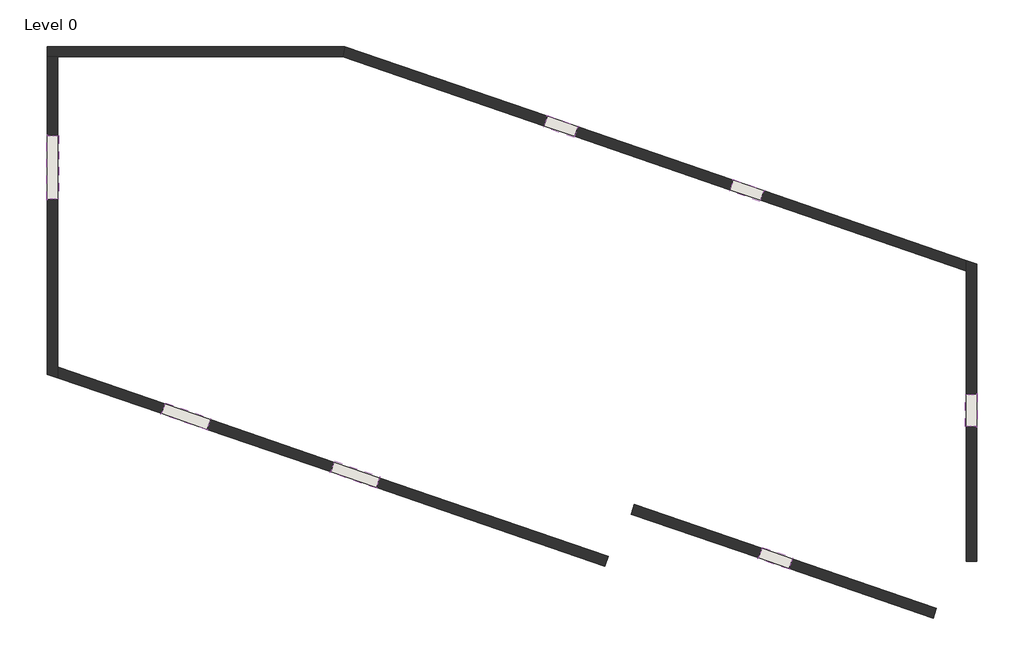
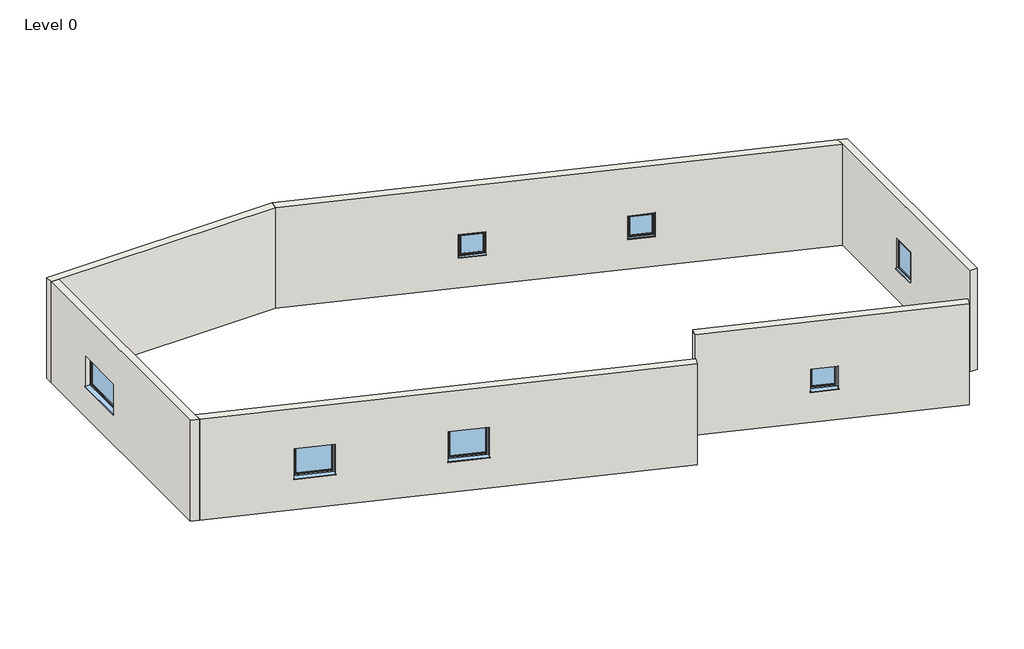
# One storey: 7 windows, 6 walls.
"""IFC4 building model written with IfcOpenShell, lengths in millimetres."""

import ifcopenshell
import ifcopenshell.guid

model = None  # the IFC model being written
_history = None  # IfcOwnerHistory: only IFC2X3 demands one
_inside = {}  # id of a spatial element -> (the spatial element, [elements in it])
_under = {}  # id of a project, library or spatial element -> (it, [spatial elements below it])
_declared = {}  # id of a project -> (the project, [libraries it declares])
_typed = {}  # id of a type object -> (the type object, [elements of that type])
_made_of = {}  # id of a material, layer set ... -> (it, [elements and type objects made of it])


def new_model(schema):
    """Start an empty IFC model of exactly this schema.

    Asked for "IFC4X3", IfcOpenShell would pick the latest addendum, in which some entities
    have other attributes; the version numbers below select the first issue.
    IFC2X3 requires an IfcOwnerHistory on every rooted entity: one is made here for all.
    """
    global model, _history
    if schema == "IFC4X3":
        model = ifcopenshell.file(schema_version=(4, 3, 0, 0))
    else:
        model = ifcopenshell.file(schema=schema)
    _inside.clear()
    _under.clear()
    _declared.clear()
    _typed.clear()
    _made_of.clear()
    _history = None
    if model.schema == "IFC2X3":
        org = make("IfcOrganization", Name="unknown")
        user = make(
            "IfcPersonAndOrganization",
            ThePerson=make("IfcPerson", FamilyName="unknown"),
            TheOrganization=org,
        )
        app = make(
            "IfcApplication",
            ApplicationDeveloper=org,
            Version="unknown",
            ApplicationFullName="unknown",
            ApplicationIdentifier="unknown",
        )
        _history = make(
            "IfcOwnerHistory",
            OwningUser=user,
            OwningApplication=app,
            ChangeAction="ADDED",
            CreationDate=0,
        )
    return model


def make(cls, **values):
    """One entity of the class cls with the attributes given. An attribute that is None is left unset."""
    return model.create_entity(
        cls, **{name: value for name, value in values.items() if value is not None}
    )


def rooted(cls, **values):
    """An entity with a GlobalId (a new one), such as an element, a storey or a relation."""
    return make(cls, GlobalId=ifcopenshell.guid.new(), OwnerHistory=_history, **values)


def si_unit(unit_type, name, prefix=None):
    """IfcSIUnit, for example si_unit("LENGTHUNIT", "METRE", prefix="MILLI")."""
    return make("IfcSIUnit", UnitType=unit_type, Prefix=prefix, Name=name)


def assignment(units):
    """IfcUnitAssignment: the units of a project."""
    return None if units is None else make("IfcUnitAssignment", Units=units)


def point(xyz):
    """IfcCartesianPoint."""
    return None if xyz is None else make("IfcCartesianPoint", Coordinates=xyz)


def direction(xyz):
    """IfcDirection."""
    return None if xyz is None else make("IfcDirection", DirectionRatios=xyz)


def frame(location, z_axis=None, x_axis=None):
    """IfcAxis2Placement3D, a coordinate frame: its origin and axes. An axis left out is left unset."""
    return make(
        "IfcAxis2Placement3D",
        Location=point(location),
        Axis=direction(z_axis),
        RefDirection=direction(x_axis),
    )


def origin():
    """The frame at (0, 0, 0) with its axes left unset."""
    return frame((0.0, 0.0, 0.0))


def place(relative_to, where):
    """IfcLocalPlacement: puts the frame where relative to a parent placement (None: the world)."""
    return make(
        "IfcLocalPlacement", PlacementRelTo=relative_to, RelativePlacement=where
    )


def context(
    kind, dimensions, precision=None, world=None, true_north=None, identifier=None
):
    """IfcGeometricRepresentationContext, for example the 3D "Model" context."""
    return make(
        "IfcGeometricRepresentationContext",
        ContextIdentifier=identifier,
        ContextType=kind,
        CoordinateSpaceDimension=dimensions,
        Precision=precision,
        WorldCoordinateSystem=world,
        TrueNorth=true_north,
    )


def project(units=None, contexts=None):
    """IfcProject with its units and contexts."""
    return rooted(
        "IfcProject",
        Name="project",
        RepresentationContexts=contexts,
        UnitsInContext=assignment(units),
    )


def spatial(cls, under=None, at=None, **own):
    """A site, building, storey or space (cls), placed at a placement, below another one or the project."""
    s = rooted(cls, ObjectPlacement=at, **own)
    if under is not None:
        _under.setdefault(under.id(), (under, []))[1].append(s)
    return s


def polyline(points):
    """IfcPolyline through the points."""
    return make("IfcPolyline", Points=[point(p) for p in points])


def outline(outer, holes=None, kind="AREA"):
    """IfcArbitraryClosedProfileDef: a profile drawn as a closed curve; with holes, ...WithVoids."""
    if holes is None:
        return make("IfcArbitraryClosedProfileDef", ProfileType=kind, OuterCurve=outer)
    return make(
        "IfcArbitraryProfileDefWithVoids",
        ProfileType=kind,
        OuterCurve=outer,
        InnerCurves=holes,
    )


def extrude(swept, where, along, depth):
    """IfcExtrudedAreaSolid: the profile swept, set in the frame where, extruded along a direction by depth."""
    return make(
        "IfcExtrudedAreaSolid",
        SweptArea=swept,
        Position=where,
        ExtrudedDirection=direction(along),
        Depth=depth,
    )


def faces_of(points, faces, orient=None, outer=None):
    """IfcFace entities. A face is a list of loops; a loop is a list of indices into points, from 0.

    orient and outer hold one flag for each loop. By default every Orientation is true, the
    first loop of a face is its IfcFaceOuterBound and the others are IfcFaceBound.
    """
    made = []
    for i, loops in enumerate(faces):
        bounds = []
        for j, loop in enumerate(loops):
            is_outer = j == 0 if outer is None else outer[i][j]
            bounds.append(
                make(
                    "IfcFaceOuterBound" if is_outer else "IfcFaceBound",
                    Bound=make("IfcPolyLoop", Polygon=[points[k] for k in loop]),
                    Orientation=True if orient is None else orient[i][j],
                )
            )
        made.append(make("IfcFace", Bounds=bounds))
    return made


def faceted_brep(points, faces, orient=None, outer=None, voids=None):
    """IfcFacetedBrep: a solid bounded by flat faces; with voids (closed shells), ...WithVoids."""
    shared = [point(p) for p in points]
    hull = make("IfcClosedShell", CfsFaces=faces_of(shared, faces, orient, outer))
    if voids is None:
        return make("IfcFacetedBrep", Outer=hull)
    return make(
        "IfcFacetedBrepWithVoids",
        Outer=hull,
        Voids=[
            make(cls, CfsFaces=faces_of(shared, fs, o, b)) for cls, fs, o, b in voids
        ],
    )


def shape(context_of_items, identifier, shape_type, items):
    """IfcShapeRepresentation: the items that make up one representation, for example the "Body"."""
    return make(
        "IfcShapeRepresentation",
        ContextOfItems=context_of_items,
        RepresentationIdentifier=identifier,
        RepresentationType=shape_type,
        Items=items,
    )


def source(mapping_origin, context_of_items, identifier, shape_type, items):
    """IfcRepresentationMap: a shape defined once, which mapped items show again and again."""
    return make(
        "IfcRepresentationMap",
        MappingOrigin=mapping_origin,
        MappedRepresentation=shape(context_of_items, identifier, shape_type, items),
    )


def transform(
    local_origin,
    x_axis=None,
    y_axis=None,
    z_axis=None,
    scale=None,
    scale2=None,
    scale3=None,
    uniform=True,
):
    """IfcCartesianTransformationOperator3D, or its non-uniform kind. x_axis, y_axis, z_axis: its Axis1, 2, 3."""
    if uniform:
        return make(
            "IfcCartesianTransformationOperator3D",
            Axis1=direction(x_axis),
            Axis2=direction(y_axis),
            LocalOrigin=point(local_origin),
            Scale=scale,
            Axis3=direction(z_axis),
        )
    return make(
        "IfcCartesianTransformationOperator3DnonUniform",
        Axis1=direction(x_axis),
        Axis2=direction(y_axis),
        LocalOrigin=point(local_origin),
        Scale=scale,
        Axis3=direction(z_axis),
        Scale2=scale2,
        Scale3=scale3,
    )


def mapped(mapping_source, mapping_target):
    """IfcMappedItem: shows the shape of a source again, moved by a transform."""
    return make(
        "IfcMappedItem", MappingSource=mapping_source, MappingTarget=mapping_target
    )


def made_of(thing, what):
    """Note that an element or type object is made of a material, layer set ...; save() writes the relation."""
    if what is not None:
        _made_of.setdefault(what.id(), (what, []))[1].append(thing)
    return thing


def element(
    cls,
    number,
    at=None,
    inside=None,
    cuts=None,
    type_object=None,
    material=None,
    context=None,
    identifier="Body",
    shape_type=None,
    held_by="IfcProductDefinitionShape",
    body=None,
    shapes=None,
    **own,
):
    """One element of the class cls, such as IfcWall. Its Tag is "e" and its number.

    at: its placement. inside: the storey or other place that contains it. cuts: it is an
    opening in that element (IfcRelVoidsElement). A single representation is given by context,
    identifier, shape_type and body (its items); several are given by shapes. held_by: the class
    of the entity that holds the representations. save() writes the other relations.
    """
    e = rooted(cls, Tag="e%d" % number, ObjectPlacement=at, **own)
    if body is not None:
        shapes = [shape(context, identifier, shape_type, body)]
    if shapes is not None:
        e.Representation = make(held_by, Representations=shapes)
    if inside is not None:
        _inside.setdefault(inside.id(), (inside, []))[1].append(e)
    if cuts is not None:
        rooted(
            "IfcRelVoidsElement", RelatingBuildingElement=cuts, RelatedOpeningElement=e
        )
    if type_object is not None:
        _typed.setdefault(type_object.id(), (type_object, []))[1].append(e)
    return made_of(e, material)


def aggregate(whole, parts):
    """IfcRelAggregates: a whole, such as a stair, and the parts it consists of."""
    return rooted("IfcRelAggregates", RelatingObject=whole, RelatedObjects=parts)


def save(model, path):
    """Write the relations noted so far, then the file.

    IfcRelAggregates (storeys below a building ...), IfcRelContainedInSpatialStructure (elements
    in a storey), IfcRelDefinesByType, IfcRelAssociatesMaterial and IfcRelDeclares: one each for
    every whole, place, type object, material and project.
    """
    for whole, parts in _under.values():
        aggregate(whole, parts)
    for where, things in _inside.values():
        rooted(
            "IfcRelContainedInSpatialStructure",
            RelatedElements=things,
            RelatingStructure=where,
        )
    for kind, things in _typed.values():
        rooted("IfcRelDefinesByType", RelatedObjects=things, RelatingType=kind)
    for what, things in _made_of.values():
        rooted("IfcRelAssociatesMaterial", RelatedObjects=things, RelatingMaterial=what)
    for by, libraries in _declared.values():
        rooted("IfcRelDeclares", RelatingContext=by, RelatedDefinitions=libraries)
    model.write(path)


def windows_sgl_plain_1360x1210mm_d0b87b97(model_context):
    return source(origin(), model_context, "Body", "SolidModel", [
        extrude(outline(polyline([(-705.0, -161.5434322), (-705.0, -136.5434322), (-680.0, -136.5434322), (-680.0, 20.4565678), (680.0, 20.4565678), (680.0, -136.5434322), (705.0, -136.5434322), (705.0, -161.5434322), (-705.0, -161.5434322)])), frame((0.0, 0.0, 900.0), z_axis=(0.0, 0.0, 1.0), x_axis=(1.0, 0.0, 0.0)), (0.0, 0.0, 1.0), 25.0),
        faceted_brep([(-680.0, 20.4565678, 900.0), (680.0, 20.4565678, 900.0), (680.0, 20.4565678, 2110.0), (-680.0, 20.4565678, 2110.0), (-620.0, 20.4565678, 2050.0), (620.0, 20.4565678, 2050.0), (620.0, 20.4565678, 975.0), (-620.0, 20.4565678, 975.0), (-680.0, 103.4565678, 2110.0), (-680.0, 103.4565678, 951.0), (-680.0, 118.4565678, 949.68767), (-680.0, 118.4565678, 944.7449676), (-680.0, 190.9565678, 933.8088847), (-680.0, 190.9565678, 900.0), (680.0, 103.4565678, 2110.0), (680.0, 103.4565678, 951.0), (-640.0, 103.4565678, 2070.0), (-640.0, 103.4565678, 963.0), (640.0, 103.4565678, 963.0), (640.0, 103.4565678, 2070.0), (-640.0, 38.4565678, 2070.0), (-640.0, 38.4565678, 963.0), (640.0, 38.4565678, 2070.0), (640.0, 38.4565678, 963.0), (-620.0, 38.4565678, 2050.0), (-620.0, 38.4565678, 975.0), (620.0, 38.4565678, 975.0), (620.0, 38.4565678, 2050.0), (680.0, 190.9565678, 900.0), (680.0, 190.9565678, 933.8088847), (680.0, 118.4565678, 944.7449676), (680.0, 118.4565678, 949.68767)], [[[0, 1, 2, 3], [4, 5, 6, 7]], [[0, 3, 8, 9, 10, 11, 12, 13]], [[9, 8, 14, 15], [16, 17, 18, 19]], [[17, 16, 20, 21]], [[20, 22, 23, 21], [24, 25, 26, 27]], [[24, 4, 7, 25]], [[3, 2, 14, 8]], [[16, 19, 22, 20]], [[5, 4, 24, 27]], [[15, 14, 2, 1, 28, 29, 30, 31]], [[19, 18, 23, 22]], [[5, 27, 26, 6]], [[28, 1, 0, 13]], [[29, 28, 13, 12]], [[30, 29, 12, 11]], [[31, 30, 11, 10]], [[15, 31, 10, 9]], [[21, 23, 18, 17]], [[7, 6, 26, 25]]]),
        extrude(outline(polyline([(610.0, 67.4565678), (-610.0, 67.4565678), (-610.0, 91.4565678), (610.0, 91.4565678), (610.0, 67.4565678)])), frame((0.0, 0.0, 993.0), z_axis=(0.0, 0.0, 1.0), x_axis=(1.0, 0.0, 0.0)), (0.0, 0.0, 1.0), 1047.0),
        faceted_brep([(-650.0, 103.4565678, 2080.0), (-650.0, 109.2300705, 2080.0), (-650.0, 109.2300705, 953.0), (-650.0, 103.4565678, 953.0), (-640.0, 38.4565678, 2070.0), (-640.0, 103.4565678, 2070.0), (-640.0, 103.4565678, 963.0), (-640.0, 38.4565678, 963.0), (-600.0, 52.9494677, 2030.0), (-610.1480377, 38.4565678, 2040.1480377), (-610.1480377, 38.4565678, 992.8519623), (-600.0, 52.9494677, 1003.0), (-600.0, 67.4565678, 2030.0), (-600.0, 67.4565678, 1003.0), (-610.0, 91.4565678, 2040.0), (-610.0, 67.4565678, 2040.0), (-610.0, 67.4565678, 993.0), (-610.0, 91.4565678, 993.0), (-600.0, 109.2300705, 2030.0), (-600.0, 91.4565678, 2030.0), (-600.0, 91.4565678, 1003.0), (-600.0, 109.2300705, 1003.0), (-617.4457548, 115.0035732, 2047.4457548), (-617.4457548, 115.0035732, 985.5542452), (-639.2153903, 115.0035732, 2069.2153903), (-639.2153903, 115.0035732, 963.7846097), (650.0, 109.2300705, 953.0), (650.0, 103.4565678, 953.0), (640.0, 103.4565678, 963.0), (640.0, 38.4565678, 963.0), (610.1480377, 38.4565678, 992.8519623), (600.0, 52.9494677, 1003.0), (600.0, 67.4565678, 1003.0), (610.0, 67.4565678, 993.0), (610.0, 91.4565678, 993.0), (600.0, 91.4565678, 1003.0), (600.0, 109.2300705, 1003.0), (617.4457548, 115.0035732, 985.5542452), (639.2153903, 115.0035732, 963.7846097), (650.0, 109.2300705, 2080.0), (650.0, 103.4565678, 2080.0), (640.0, 103.4565678, 2070.0), (640.0, 38.4565678, 2070.0), (610.1480377, 38.4565678, 2040.1480377), (600.0, 52.9494677, 2030.0), (600.0, 67.4565678, 2030.0), (610.0, 67.4565678, 2040.0), (610.0, 91.4565678, 2040.0), (600.0, 91.4565678, 2030.0), (600.0, 109.2300705, 2030.0), (617.4457548, 115.0035732, 2047.4457548), (639.2153903, 115.0035732, 2069.2153903)], [[[0, 1, 2, 3]], [[4, 5, 6, 7]], [[8, 9, 10, 11]], [[12, 8, 11, 13]], [[14, 15, 16, 17]], [[18, 19, 20, 21]], [[22, 18, 21, 23]], [[1, 24, 25, 2]], [[3, 2, 26, 27]], [[7, 6, 28, 29]], [[11, 10, 30, 31]], [[13, 11, 31, 32]], [[17, 16, 33, 34]], [[21, 20, 35, 36]], [[23, 21, 36, 37]], [[2, 25, 38, 26]], [[27, 26, 39, 40]], [[29, 28, 41, 42]], [[31, 30, 43, 44]], [[32, 31, 44, 45]], [[34, 33, 46, 47]], [[36, 35, 48, 49]], [[37, 36, 49, 50]], [[26, 38, 51, 39]], [[40, 39, 1, 0]], [[3, 27, 40, 0], [5, 41, 28, 6]], [[42, 41, 5, 4]], [[7, 29, 42, 4], [9, 43, 30, 10]], [[44, 43, 9, 8]], [[45, 44, 8, 12]], [[15, 46, 33, 16], [13, 32, 45, 12]], [[47, 46, 15, 14]], [[17, 34, 47, 14], [19, 48, 35, 20]], [[49, 48, 19, 18]], [[50, 49, 18, 22]], [[24, 51, 38, 25], [23, 37, 50, 22]], [[39, 51, 24, 1]]]),
    ])


def windows_sgl_plain_1810x1210mm_114720e4(model_context):
    return source(origin(), model_context, "Body", "SolidModel", [
        extrude(outline(polyline([(-930.0, -161.5434322), (-930.0, -136.5434322), (-905.0, -136.5434322), (-905.0, 20.4565678), (905.0, 20.4565678), (905.0, -136.5434322), (930.0, -136.5434322), (930.0, -161.5434322), (-930.0, -161.5434322)])), frame((0.0, 0.0, 900.0), z_axis=(0.0, 0.0, 1.0), x_axis=(1.0, 0.0, 0.0)), (0.0, 0.0, 1.0), 25.0),
        faceted_brep([(-905.0, 20.4565678, 900.0), (905.0, 20.4565678, 900.0), (905.0, 20.4565678, 2110.0), (-905.0, 20.4565678, 2110.0), (-845.0, 20.4565678, 2050.0), (845.0, 20.4565678, 2050.0), (845.0, 20.4565678, 975.0), (-845.0, 20.4565678, 975.0), (-905.0, 103.4565678, 2110.0), (-905.0, 103.4565678, 951.0), (-905.0, 118.4565678, 949.68767), (-905.0, 118.4565678, 944.7449676), (-905.0, 190.9565678, 933.8088847), (-905.0, 190.9565678, 900.0), (905.0, 103.4565678, 2110.0), (905.0, 103.4565678, 951.0), (-865.0, 103.4565678, 2070.0), (-865.0, 103.4565678, 963.0), (865.0, 103.4565678, 963.0), (865.0, 103.4565678, 2070.0), (-865.0, 38.4565678, 2070.0), (-865.0, 38.4565678, 963.0), (865.0, 38.4565678, 2070.0), (865.0, 38.4565678, 963.0), (-845.0, 38.4565678, 2050.0), (-845.0, 38.4565678, 975.0), (845.0, 38.4565678, 975.0), (845.0, 38.4565678, 2050.0), (905.0, 190.9565678, 900.0), (905.0, 190.9565678, 933.8088847), (905.0, 118.4565678, 944.7449676), (905.0, 118.4565678, 949.68767)], [[[0, 1, 2, 3], [4, 5, 6, 7]], [[0, 3, 8, 9, 10, 11, 12, 13]], [[9, 8, 14, 15], [16, 17, 18, 19]], [[17, 16, 20, 21]], [[20, 22, 23, 21], [24, 25, 26, 27]], [[24, 4, 7, 25]], [[3, 2, 14, 8]], [[16, 19, 22, 20]], [[5, 4, 24, 27]], [[15, 14, 2, 1, 28, 29, 30, 31]], [[19, 18, 23, 22]], [[5, 27, 26, 6]], [[28, 1, 0, 13]], [[29, 28, 13, 12]], [[30, 29, 12, 11]], [[31, 30, 11, 10]], [[15, 31, 10, 9]], [[21, 23, 18, 17]], [[7, 6, 26, 25]]]),
        extrude(outline(polyline([(835.0, 67.4565678), (-835.0, 67.4565678), (-835.0, 91.4565678), (835.0, 91.4565678), (835.0, 67.4565678)])), frame((0.0, 0.0, 993.0), z_axis=(0.0, 0.0, 1.0), x_axis=(1.0, 0.0, 0.0)), (0.0, 0.0, 1.0), 1047.0),
        faceted_brep([(-875.0, 103.4565678, 2080.0), (-875.0, 109.2300705, 2080.0), (-875.0, 109.2300705, 953.0), (-875.0, 103.4565678, 953.0), (-865.0, 38.4565678, 2070.0), (-865.0, 103.4565678, 2070.0), (-865.0, 103.4565678, 963.0), (-865.0, 38.4565678, 963.0), (-825.0, 52.9494677, 2030.0), (-835.1480377, 38.4565678, 2040.1480377), (-835.1480377, 38.4565678, 992.8519623), (-825.0, 52.9494677, 1003.0), (-825.0, 67.4565678, 2030.0), (-825.0, 67.4565678, 1003.0), (-835.0, 91.4565678, 2040.0), (-835.0, 67.4565678, 2040.0), (-835.0, 67.4565678, 993.0), (-835.0, 91.4565678, 993.0), (-825.0, 109.2300705, 2030.0), (-825.0, 91.4565678, 2030.0), (-825.0, 91.4565678, 1003.0), (-825.0, 109.2300705, 1003.0), (-842.4457548, 115.0035732, 2047.4457548), (-842.4457548, 115.0035732, 985.5542452), (-864.2153903, 115.0035732, 2069.2153903), (-864.2153903, 115.0035732, 963.7846097), (875.0, 109.2300705, 953.0), (875.0, 103.4565678, 953.0), (865.0, 103.4565678, 963.0), (865.0, 38.4565678, 963.0), (835.1480377, 38.4565678, 992.8519623), (825.0, 52.9494677, 1003.0), (825.0, 67.4565678, 1003.0), (835.0, 67.4565678, 993.0), (835.0, 91.4565678, 993.0), (825.0, 91.4565678, 1003.0), (825.0, 109.2300705, 1003.0), (842.4457548, 115.0035732, 985.5542452), (864.2153903, 115.0035732, 963.7846097), (875.0, 109.2300705, 2080.0), (875.0, 103.4565678, 2080.0), (865.0, 103.4565678, 2070.0), (865.0, 38.4565678, 2070.0), (835.1480377, 38.4565678, 2040.1480377), (825.0, 52.9494677, 2030.0), (825.0, 67.4565678, 2030.0), (835.0, 67.4565678, 2040.0), (835.0, 91.4565678, 2040.0), (825.0, 91.4565678, 2030.0), (825.0, 109.2300705, 2030.0), (842.4457548, 115.0035732, 2047.4457548), (864.2153903, 115.0035732, 2069.2153903)], [[[0, 1, 2, 3]], [[4, 5, 6, 7]], [[8, 9, 10, 11]], [[12, 8, 11, 13]], [[14, 15, 16, 17]], [[18, 19, 20, 21]], [[22, 18, 21, 23]], [[1, 24, 25, 2]], [[3, 2, 26, 27]], [[7, 6, 28, 29]], [[11, 10, 30, 31]], [[13, 11, 31, 32]], [[17, 16, 33, 34]], [[21, 20, 35, 36]], [[23, 21, 36, 37]], [[2, 25, 38, 26]], [[27, 26, 39, 40]], [[29, 28, 41, 42]], [[31, 30, 43, 44]], [[32, 31, 44, 45]], [[34, 33, 46, 47]], [[36, 35, 48, 49]], [[37, 36, 49, 50]], [[26, 38, 51, 39]], [[40, 39, 1, 0]], [[3, 27, 40, 0], [5, 41, 28, 6]], [[42, 41, 5, 4]], [[7, 29, 42, 4], [9, 43, 30, 10]], [[44, 43, 9, 8]], [[45, 44, 8, 12]], [[15, 46, 33, 16], [13, 32, 45, 12]], [[47, 46, 15, 14]], [[17, 34, 47, 14], [19, 48, 35, 20]], [[49, 48, 19, 18]], [[50, 49, 18, 22]], [[24, 51, 38, 25], [23, 37, 50, 22]], [[39, 51, 24, 1]]]),
    ])


def windows_sgl_plain_910x1210mm_58c8e711(model_context):
    return source(origin(), model_context, "Body", "SolidModel", [
        extrude(outline(polyline([(-480.0, -161.5434322), (-480.0, -136.5434322), (-455.0, -136.5434322), (-455.0, 20.4565678), (455.0, 20.4565678), (455.0, -136.5434322), (480.0, -136.5434322), (480.0, -161.5434322), (-480.0, -161.5434322)])), frame((0.0, 0.0, 900.0), z_axis=(0.0, 0.0, 1.0), x_axis=(1.0, 0.0, 0.0)), (0.0, 0.0, 1.0), 25.0),
        faceted_brep([(-455.0, 20.4565678, 900.0), (455.0, 20.4565678, 900.0), (455.0, 20.4565678, 2110.0), (-455.0, 20.4565678, 2110.0), (-395.0, 20.4565678, 2050.0), (395.0, 20.4565678, 2050.0), (395.0, 20.4565678, 975.0), (-395.0, 20.4565678, 975.0), (-455.0, 103.4565678, 2110.0), (-455.0, 103.4565678, 951.0), (-455.0, 118.4565678, 949.68767), (-455.0, 118.4565678, 944.7449676), (-455.0, 190.9565678, 933.8088847), (-455.0, 190.9565678, 900.0), (455.0, 103.4565678, 2110.0), (455.0, 103.4565678, 951.0), (-415.0, 103.4565678, 2070.0), (-415.0, 103.4565678, 963.0), (415.0, 103.4565678, 963.0), (415.0, 103.4565678, 2070.0), (-415.0, 38.4565678, 2070.0), (-415.0, 38.4565678, 963.0), (415.0, 38.4565678, 2070.0), (415.0, 38.4565678, 963.0), (-395.0, 38.4565678, 2050.0), (-395.0, 38.4565678, 975.0), (395.0, 38.4565678, 975.0), (395.0, 38.4565678, 2050.0), (455.0, 190.9565678, 900.0), (455.0, 190.9565678, 933.8088847), (455.0, 118.4565678, 944.7449676), (455.0, 118.4565678, 949.68767)], [[[0, 1, 2, 3], [4, 5, 6, 7]], [[0, 3, 8, 9, 10, 11, 12, 13]], [[9, 8, 14, 15], [16, 17, 18, 19]], [[17, 16, 20, 21]], [[20, 22, 23, 21], [24, 25, 26, 27]], [[24, 4, 7, 25]], [[3, 2, 14, 8]], [[16, 19, 22, 20]], [[5, 4, 24, 27]], [[15, 14, 2, 1, 28, 29, 30, 31]], [[19, 18, 23, 22]], [[5, 27, 26, 6]], [[28, 1, 0, 13]], [[29, 28, 13, 12]], [[30, 29, 12, 11]], [[31, 30, 11, 10]], [[15, 31, 10, 9]], [[21, 23, 18, 17]], [[7, 6, 26, 25]]]),
        extrude(outline(polyline([(385.0, 67.4565678), (-385.0, 67.4565678), (-385.0, 91.4565678), (385.0, 91.4565678), (385.0, 67.4565678)])), frame((0.0, 0.0, 993.0), z_axis=(0.0, 0.0, 1.0), x_axis=(1.0, 0.0, 0.0)), (0.0, 0.0, 1.0), 1047.0),
        faceted_brep([(-425.0, 103.4565678, 2080.0), (-425.0, 109.2300705, 2080.0), (-425.0, 109.2300705, 953.0), (-425.0, 103.4565678, 953.0), (-415.0, 38.4565678, 2070.0), (-415.0, 103.4565678, 2070.0), (-415.0, 103.4565678, 963.0), (-415.0, 38.4565678, 963.0), (-375.0, 52.9494677, 2030.0), (-385.1480377, 38.4565678, 2040.1480377), (-385.1480377, 38.4565678, 992.8519623), (-375.0, 52.9494677, 1003.0), (-375.0, 67.4565678, 2030.0), (-375.0, 67.4565678, 1003.0), (-385.0, 91.4565678, 2040.0), (-385.0, 67.4565678, 2040.0), (-385.0, 67.4565678, 993.0), (-385.0, 91.4565678, 993.0), (-375.0, 109.2300705, 2030.0), (-375.0, 91.4565678, 2030.0), (-375.0, 91.4565678, 1003.0), (-375.0, 109.2300705, 1003.0), (-392.4457548, 115.0035732, 2047.4457548), (-392.4457548, 115.0035732, 985.5542452), (-414.2153903, 115.0035732, 2069.2153903), (-414.2153903, 115.0035732, 963.7846097), (425.0, 109.2300705, 953.0), (425.0, 103.4565678, 953.0), (415.0, 103.4565678, 963.0), (415.0, 38.4565678, 963.0), (385.1480377, 38.4565678, 992.8519623), (375.0, 52.9494677, 1003.0), (375.0, 67.4565678, 1003.0), (385.0, 67.4565678, 993.0), (385.0, 91.4565678, 993.0), (375.0, 91.4565678, 1003.0), (375.0, 109.2300705, 1003.0), (392.4457548, 115.0035732, 985.5542452), (414.2153903, 115.0035732, 963.7846097), (425.0, 109.2300705, 2080.0), (425.0, 103.4565678, 2080.0), (415.0, 103.4565678, 2070.0), (415.0, 38.4565678, 2070.0), (385.1480377, 38.4565678, 2040.1480377), (375.0, 52.9494677, 2030.0), (375.0, 67.4565678, 2030.0), (385.0, 67.4565678, 2040.0), (385.0, 91.4565678, 2040.0), (375.0, 91.4565678, 2030.0), (375.0, 109.2300705, 2030.0), (392.4457548, 115.0035732, 2047.4457548), (414.2153903, 115.0035732, 2069.2153903)], [[[0, 1, 2, 3]], [[4, 5, 6, 7]], [[8, 9, 10, 11]], [[12, 8, 11, 13]], [[14, 15, 16, 17]], [[18, 19, 20, 21]], [[22, 18, 21, 23]], [[1, 24, 25, 2]], [[3, 2, 26, 27]], [[7, 6, 28, 29]], [[11, 10, 30, 31]], [[13, 11, 31, 32]], [[17, 16, 33, 34]], [[21, 20, 35, 36]], [[23, 21, 36, 37]], [[2, 25, 38, 26]], [[27, 26, 39, 40]], [[29, 28, 41, 42]], [[31, 30, 43, 44]], [[32, 31, 44, 45]], [[34, 33, 46, 47]], [[36, 35, 48, 49]], [[37, 36, 49, 50]], [[26, 38, 51, 39]], [[40, 39, 1, 0]], [[3, 27, 40, 0], [5, 41, 28, 6]], [[42, 41, 5, 4]], [[7, 29, 42, 4], [9, 43, 30, 10]], [[44, 43, 9, 8]], [[45, 44, 8, 12]], [[15, 46, 33, 16], [13, 32, 45, 12]], [[47, 46, 15, 14]], [[17, 34, 47, 14], [19, 48, 35, 20]], [[49, 48, 19, 18]], [[50, 49, 18, 22]], [[24, 51, 38, 25], [23, 37, 50, 22]], [[39, 51, 24, 1]]]),
    ])


def windows_sgl_plain_910x910mm_b9caa461(model_context):
    return source(origin(), model_context, "Body", "SolidModel", [
        extrude(outline(polyline([(-480.0, -161.5434322), (-480.0, -136.5434322), (-455.0, -136.5434322), (-455.0, 20.4565678), (455.0, 20.4565678), (455.0, -136.5434322), (480.0, -136.5434322), (480.0, -161.5434322), (-480.0, -161.5434322)])), frame((0.0, 0.0, 1200.0), z_axis=(0.0, 0.0, 1.0), x_axis=(1.0, 0.0, 0.0)), (0.0, 0.0, 1.0), 25.0),
        faceted_brep([(-455.0, 20.4565678, 1200.0), (455.0, 20.4565678, 1200.0), (455.0, 20.4565678, 2110.0), (-455.0, 20.4565678, 2110.0), (-395.0, 20.4565678, 2050.0), (395.0, 20.4565678, 2050.0), (395.0, 20.4565678, 1275.0), (-395.0, 20.4565678, 1275.0), (-455.0, 103.4565678, 2110.0), (-455.0, 103.4565678, 1251.0), (-455.0, 118.4565678, 1249.68767), (-455.0, 118.4565678, 1244.7449676), (-455.0, 190.9565678, 1233.8088847), (-455.0, 190.9565678, 1200.0), (455.0, 103.4565678, 2110.0), (455.0, 103.4565678, 1251.0), (-415.0, 103.4565678, 2070.0), (-415.0, 103.4565678, 1263.0), (415.0, 103.4565678, 1263.0), (415.0, 103.4565678, 2070.0), (-415.0, 38.4565678, 2070.0), (-415.0, 38.4565678, 1263.0), (415.0, 38.4565678, 2070.0), (415.0, 38.4565678, 1263.0), (-395.0, 38.4565678, 2050.0), (-395.0, 38.4565678, 1275.0), (395.0, 38.4565678, 1275.0), (395.0, 38.4565678, 2050.0), (455.0, 190.9565678, 1200.0), (455.0, 190.9565678, 1233.8088847), (455.0, 118.4565678, 1244.7449676), (455.0, 118.4565678, 1249.68767)], [[[0, 1, 2, 3], [4, 5, 6, 7]], [[0, 3, 8, 9, 10, 11, 12, 13]], [[9, 8, 14, 15], [16, 17, 18, 19]], [[17, 16, 20, 21]], [[20, 22, 23, 21], [24, 25, 26, 27]], [[24, 4, 7, 25]], [[3, 2, 14, 8]], [[16, 19, 22, 20]], [[5, 4, 24, 27]], [[15, 14, 2, 1, 28, 29, 30, 31]], [[19, 18, 23, 22]], [[5, 27, 26, 6]], [[28, 1, 0, 13]], [[29, 28, 13, 12]], [[30, 29, 12, 11]], [[31, 30, 11, 10]], [[15, 31, 10, 9]], [[21, 23, 18, 17]], [[7, 6, 26, 25]]]),
        extrude(outline(polyline([(385.0, 67.4565678), (-385.0, 67.4565678), (-385.0, 91.4565678), (385.0, 91.4565678), (385.0, 67.4565678)])), frame((0.0, 0.0, 1293.0), z_axis=(0.0, 0.0, 1.0), x_axis=(1.0, 0.0, 0.0)), (0.0, 0.0, 1.0), 747.0),
        faceted_brep([(-425.0, 103.4565678, 2080.0), (-425.0, 109.2300705, 2080.0), (-425.0, 109.2300705, 1253.0), (-425.0, 103.4565678, 1253.0), (-415.0, 38.4565678, 2070.0), (-415.0, 103.4565678, 2070.0), (-415.0, 103.4565678, 1263.0), (-415.0, 38.4565678, 1263.0), (-375.0, 52.9494677, 2030.0), (-385.1480377, 38.4565678, 2040.1480377), (-385.1480377, 38.4565678, 1292.8519623), (-375.0, 52.9494677, 1303.0), (-375.0, 67.4565678, 2030.0), (-375.0, 67.4565678, 1303.0), (-385.0, 91.4565678, 2040.0), (-385.0, 67.4565678, 2040.0), (-385.0, 67.4565678, 1293.0), (-385.0, 91.4565678, 1293.0), (-375.0, 109.2300705, 2030.0), (-375.0, 91.4565678, 2030.0), (-375.0, 91.4565678, 1303.0), (-375.0, 109.2300705, 1303.0), (-392.4457548, 115.0035732, 2047.4457548), (-392.4457548, 115.0035732, 1285.5542452), (-414.2153903, 115.0035732, 2069.2153903), (-414.2153903, 115.0035732, 1263.7846097), (425.0, 109.2300705, 1253.0), (425.0, 103.4565678, 1253.0), (415.0, 103.4565678, 1263.0), (415.0, 38.4565678, 1263.0), (385.1480377, 38.4565678, 1292.8519623), (375.0, 52.9494677, 1303.0), (375.0, 67.4565678, 1303.0), (385.0, 67.4565678, 1293.0), (385.0, 91.4565678, 1293.0), (375.0, 91.4565678, 1303.0), (375.0, 109.2300705, 1303.0), (392.4457548, 115.0035732, 1285.5542452), (414.2153903, 115.0035732, 1263.7846097), (425.0, 109.2300705, 2080.0), (425.0, 103.4565678, 2080.0), (415.0, 103.4565678, 2070.0), (415.0, 38.4565678, 2070.0), (385.1480377, 38.4565678, 2040.1480377), (375.0, 52.9494677, 2030.0), (375.0, 67.4565678, 2030.0), (385.0, 67.4565678, 2040.0), (385.0, 91.4565678, 2040.0), (375.0, 91.4565678, 2030.0), (375.0, 109.2300705, 2030.0), (392.4457548, 115.0035732, 2047.4457548), (414.2153903, 115.0035732, 2069.2153903)], [[[0, 1, 2, 3]], [[4, 5, 6, 7]], [[8, 9, 10, 11]], [[12, 8, 11, 13]], [[14, 15, 16, 17]], [[18, 19, 20, 21]], [[22, 18, 21, 23]], [[1, 24, 25, 2]], [[3, 2, 26, 27]], [[7, 6, 28, 29]], [[11, 10, 30, 31]], [[13, 11, 31, 32]], [[17, 16, 33, 34]], [[21, 20, 35, 36]], [[23, 21, 36, 37]], [[2, 25, 38, 26]], [[27, 26, 39, 40]], [[29, 28, 41, 42]], [[31, 30, 43, 44]], [[32, 31, 44, 45]], [[34, 33, 46, 47]], [[36, 35, 48, 49]], [[37, 36, 49, 50]], [[26, 38, 51, 39]], [[40, 39, 1, 0]], [[3, 27, 40, 0], [5, 41, 28, 6]], [[42, 41, 5, 4]], [[7, 29, 42, 4], [9, 43, 30, 10]], [[44, 43, 9, 8]], [[45, 44, 8, 12]], [[15, 46, 33, 16], [13, 32, 45, 12]], [[47, 46, 15, 14]], [[17, 34, 47, 14], [19, 48, 35, 20]], [[49, 48, 19, 18]], [[50, 49, 18, 22]], [[24, 51, 38, 25], [23, 37, 50, 22]], [[39, 51, 24, 1]]]),
    ])


def windows_sgl_plain_910x910mm_91039d7f(model_context):
    return source(origin(), model_context, "Body", "SolidModel", [
        extrude(outline(polyline([(-480.0, 161.5434322), (480.0, 161.5434322), (480.0, 136.5434322), (455.0, 136.5434322), (455.0, -20.4565678), (-455.0, -20.4565678), (-455.0, 136.5434322), (-480.0, 136.5434322), (-480.0, 161.5434322)])), frame((0.0, 0.0, 1200.0), z_axis=(0.0, 0.0, 1.0), x_axis=(1.0, 0.0, 0.0)), (0.0, 0.0, 1.0), 25.0),
        faceted_brep([(-455.0, -20.4565678, 1200.0), (-455.0, -20.4565678, 2110.0), (455.0, -20.4565678, 2110.0), (455.0, -20.4565678, 1200.0), (-395.0, -20.4565678, 2050.0), (-395.0, -20.4565678, 1275.0), (395.0, -20.4565678, 1275.0), (395.0, -20.4565678, 2050.0), (-455.0, -190.9565678, 1200.0), (-455.0, -190.9565678, 1233.8088847), (-455.0, -118.4565678, 1244.7449676), (-455.0, -118.4565678, 1249.68767), (-455.0, -103.4565678, 1251.0), (-455.0, -103.4565678, 2110.0), (455.0, -103.4565678, 1251.0), (455.0, -103.4565678, 2110.0), (-415.0, -103.4565678, 2070.0), (415.0, -103.4565678, 2070.0), (415.0, -103.4565678, 1263.0), (-415.0, -103.4565678, 1263.0), (-415.0, -38.4565678, 1263.0), (-415.0, -38.4565678, 2070.0), (415.0, -38.4565678, 1263.0), (415.0, -38.4565678, 2070.0), (-395.0, -38.4565678, 2050.0), (395.0, -38.4565678, 2050.0), (395.0, -38.4565678, 1275.0), (-395.0, -38.4565678, 1275.0), (455.0, -118.4565678, 1249.68767), (455.0, -118.4565678, 1244.7449676), (455.0, -190.9565678, 1233.8088847), (455.0, -190.9565678, 1200.0)], [[[0, 1, 2, 3], [4, 5, 6, 7]], [[0, 8, 9, 10, 11, 12, 13, 1]], [[12, 14, 15, 13], [16, 17, 18, 19]], [[19, 20, 21, 16]], [[21, 20, 22, 23], [24, 25, 26, 27]], [[24, 27, 5, 4]], [[1, 13, 15, 2]], [[16, 21, 23, 17]], [[7, 25, 24, 4]], [[14, 28, 29, 30, 31, 3, 2, 15]], [[17, 23, 22, 18]], [[7, 6, 26, 25]], [[31, 8, 0, 3]], [[30, 9, 8, 31]], [[29, 10, 9, 30]], [[28, 11, 10, 29]], [[14, 12, 11, 28]], [[20, 19, 18, 22]], [[5, 27, 26, 6]]]),
        extrude(outline(polyline([(385.0, -67.4565678), (385.0, -91.4565678), (-385.0, -91.4565678), (-385.0, -67.4565678), (385.0, -67.4565678)])), frame((0.0, 0.0, 1293.0), z_axis=(0.0, 0.0, 1.0), x_axis=(1.0, 0.0, 0.0)), (0.0, 0.0, 1.0), 747.0),
        faceted_brep([(-425.0, -103.4565678, 2080.0), (-425.0, -103.4565678, 1253.0), (-425.0, -109.2300705, 1253.0), (-425.0, -109.2300705, 2080.0), (-415.0, -38.4565678, 2070.0), (-415.0, -38.4565678, 1263.0), (-415.0, -103.4565678, 1263.0), (-415.0, -103.4565678, 2070.0), (-375.0, -52.9494677, 2030.0), (-375.0, -52.9494677, 1303.0), (-385.1480377, -38.4565678, 1292.8519623), (-385.1480377, -38.4565678, 2040.1480377), (-375.0, -67.4565678, 2030.0), (-375.0, -67.4565678, 1303.0), (-385.0, -91.4565678, 2040.0), (-385.0, -91.4565678, 1293.0), (-385.0, -67.4565678, 1293.0), (-385.0, -67.4565678, 2040.0), (-375.0, -109.2300705, 2030.0), (-375.0, -109.2300705, 1303.0), (-375.0, -91.4565678, 1303.0), (-375.0, -91.4565678, 2030.0), (-392.4457548, -115.0035732, 2047.4457548), (-392.4457548, -115.0035732, 1285.5542452), (-414.2153903, -115.0035732, 1263.7846097), (-414.2153903, -115.0035732, 2069.2153903), (425.0, -103.4565678, 1253.0), (425.0, -109.2300705, 1253.0), (415.0, -38.4565678, 1263.0), (415.0, -103.4565678, 1263.0), (375.0, -52.9494677, 1303.0), (385.1480377, -38.4565678, 1292.8519623), (375.0, -67.4565678, 1303.0), (385.0, -91.4565678, 1293.0), (385.0, -67.4565678, 1293.0), (375.0, -109.2300705, 1303.0), (375.0, -91.4565678, 1303.0), (392.4457548, -115.0035732, 1285.5542452), (414.2153903, -115.0035732, 1263.7846097), (425.0, -103.4565678, 2080.0), (425.0, -109.2300705, 2080.0), (415.0, -38.4565678, 2070.0), (415.0, -103.4565678, 2070.0), (375.0, -52.9494677, 2030.0), (385.1480377, -38.4565678, 2040.1480377), (375.0, -67.4565678, 2030.0), (385.0, -91.4565678, 2040.0), (385.0, -67.4565678, 2040.0), (375.0, -109.2300705, 2030.0), (375.0, -91.4565678, 2030.0), (392.4457548, -115.0035732, 2047.4457548), (414.2153903, -115.0035732, 2069.2153903)], [[[0, 1, 2, 3]], [[4, 5, 6, 7]], [[8, 9, 10, 11]], [[12, 13, 9, 8]], [[14, 15, 16, 17]], [[18, 19, 20, 21]], [[22, 23, 19, 18]], [[3, 2, 24, 25]], [[1, 26, 27, 2]], [[5, 28, 29, 6]], [[9, 30, 31, 10]], [[13, 32, 30, 9]], [[15, 33, 34, 16]], [[19, 35, 36, 20]], [[23, 37, 35, 19]], [[2, 27, 38, 24]], [[26, 39, 40, 27]], [[28, 41, 42, 29]], [[30, 43, 44, 31]], [[32, 45, 43, 30]], [[33, 46, 47, 34]], [[35, 48, 49, 36]], [[37, 50, 48, 35]], [[27, 40, 51, 38]], [[39, 0, 3, 40]], [[1, 0, 39, 26], [7, 6, 29, 42]], [[41, 4, 7, 42]], [[5, 4, 41, 28], [11, 10, 31, 44]], [[43, 8, 11, 44]], [[45, 12, 8, 43]], [[17, 16, 34, 47], [13, 12, 45, 32]], [[46, 14, 17, 47]], [[15, 14, 46, 33], [21, 20, 36, 49]], [[48, 18, 21, 49]], [[50, 22, 18, 48]], [[25, 24, 38, 51], [23, 22, 50, 37]], [[40, 3, 25, 51]]]),
    ])


model = new_model("IFC4")

# Units and contexts
model_context = context("Model", 3, world=origin())
ifc_project = project(units=[si_unit("LENGTHUNIT", "METRE", prefix="MILLI")], contexts=[model_context])

# Site, building, storey
site = spatial("IfcSite", under=ifc_project)
building = spatial("IfcBuilding", under=site)
storey = spatial("IfcBuildingStorey", under=building, Name="Level 0", Elevation=0.0)

# Walls
placement = place(None, origin())
element("IfcWall", 1, ObjectType="Wall-Ext_102Bwk-75Ins-100LBlk-12P", at=placement, inside=storey, context=model_context, shape_type="Brep", body=[
    faceted_brep([(-7959.4403651, 3140.4215611, 0.0), (9809.9845257, -2978.0821011, 0.0), (9809.9845257, -2978.0821011, 4000.0), (-7959.4403651, 3140.4215611, 4000.0), (-1359.0254471, 867.7164457, 2110.0), (-1359.0254471, 867.7164457, 1200.0), (-2219.4473509, 1163.9834663, 1200.0), (-2219.4473509, 1163.9834663, 2110.0), (3935.8785762, -955.4652193, 2110.0), (3935.8785762, -955.4652193, 1200.0), (3075.4566724, -659.1981987, 1200.0), (3075.4566724, -659.1981987, 2110.0), (-7910.9110085, 3430.4215611, 0.0), (-7910.9110085, 3430.4215611, 4000.0), (9809.9845257, -2671.3721035, 4000.0), (9809.9845257, -2671.3721035, 0.0), (-1264.6106823, 1141.9168326, 2110.0), (-2125.0325861, 1438.1838532, 2110.0), (-2125.0325861, 1438.1838532, 1200.0), (-1264.6106823, 1141.9168326, 1200.0), (4030.293341, -681.2648323, 2110.0), (3169.8714372, -384.9978118, 2110.0), (3169.8714372, -384.9978118, 1200.0), (4030.293341, -681.2648323, 1200.0)], [[[0, 1, 2, 3], [4, 5, 6, 7], [8, 9, 10, 11]], [[12, 13, 14, 15], [16, 17, 18, 19], [20, 21, 22, 23]], [[1, 0, 12, 15]], [[3, 2, 14, 13]], [[5, 4, 16, 19]], [[6, 5, 19, 18]], [[7, 6, 18, 17]], [[4, 7, 17, 16]], [[0, 3, 13, 12]], [[2, 1, 15, 14]], [[9, 8, 20, 23]], [[10, 9, 23, 22]], [[11, 10, 22, 21]], [[8, 11, 21, 20]]]),
])
element("IfcWall", 2, ObjectType="Wall-Ext_102Bwk-75Ins-100LBlk-12P", at=placement, inside=storey, context=model_context, shape_type="Brep", body=[
    faceted_brep([(-7910.9110085, 3430.4215611, 0.0), (-16380.1756868, 3430.4215611, 0.0), (-16380.1756868, 3430.4215611, 4000.0), (-7910.9110085, 3430.4215611, 4000.0), (-7959.4403651, 3140.4215611, 0.0), (-7959.4403651, 3140.4215611, 4000.0), (-16090.1756868, 3140.4215611, 4000.0), (-16380.1756868, 3140.4215611, 4000.0), (-16380.1756868, 3140.4215611, 0.0), (-16090.1756868, 3140.4215611, 0.0)], [[[0, 1, 2, 3]], [[4, 5, 6, 7, 8, 9]], [[1, 0, 4, 9, 8]], [[3, 2, 7, 6, 5]], [[0, 3, 5, 4]], [[2, 1, 8, 7]]]),
])
element("IfcWall", 3, ObjectType="Wall-Ext_102Bwk-75Ins-100LBlk-12P", at=placement, inside=storey, context=model_context, shape_type="Brep", body=[
    faceted_brep([(-16380.1756868, 3140.4215611, 0.0), (-16380.1756868, -5918.0059337, 0.0), (-16380.1756868, -5918.0059337, 4000.0), (-16380.1756868, 3140.4215611, 4000.0), (-16380.1756868, 890.4215611, 2410.0), (-16380.1756868, -919.5784389, 2410.0), (-16380.1756868, -919.5784389, 1200.0), (-16380.1756868, 890.4215611, 1200.0), (-16090.1756868, 3140.4215611, 0.0), (-16090.1756868, 3140.4215611, 4000.0), (-16090.1756868, -5711.150944, 4000.0), (-16090.1756868, -6017.8609416, 4000.0), (-16090.1756868, -6017.8609416, 0.0), (-16090.1756868, -5711.150944, 0.0), (-16090.1756868, 890.4215611, 2410.0), (-16090.1756868, 890.4215611, 1200.0), (-16090.1756868, -919.5784389, 1200.0), (-16090.1756868, -919.5784389, 2410.0)], [[[0, 1, 2, 3], [4, 5, 6, 7]], [[8, 9, 10, 11, 12, 13], [14, 15, 16, 17]], [[1, 0, 8, 13, 12]], [[3, 2, 11, 10, 9]], [[0, 3, 9, 8]], [[2, 1, 12, 11]], [[15, 14, 4, 7]], [[16, 15, 7, 6]], [[17, 16, 6, 5]], [[14, 17, 5, 4]]]),
])
element("IfcWall", 4, ObjectType="Wall-Ext_102Bwk-75Ins-100LBlk-12P", at=placement, inside=storey, context=model_context, shape_type="Brep", body=[
    faceted_brep([(-16090.1756868, -6017.8609416, 0.0), (-492.2228567, -11388.6668118, 0.0), (-492.2228567, -11388.6668118, 4000.0), (-16090.1756868, -6017.8609416, 4000.0), (-8296.6382472, -8701.3910872, 2410.0), (-7010.7329844, -9144.1637773, 2410.0), (-7010.7329844, -9144.1637773, 1200.0), (-8296.6382472, -8701.3910872, 1200.0), (-13118.7829828, -7040.9934995, 2410.0), (-11832.87772, -7483.7661896, 2410.0), (-11832.87772, -7483.7661896, 1200.0), (-13118.7829828, -7040.9934995, 1200.0), (-16090.1756868, -5711.150944, 0.0), (-16090.1756868, -5711.150944, 4000.0), (-397.8080919, -11114.4664248, 4000.0), (-397.8080919, -11114.4664248, 0.0), (-8202.2234824, -8427.1907003, 2410.0), (-8202.2234824, -8427.1907003, 1200.0), (-6916.3182196, -8869.9633904, 1200.0), (-6916.3182196, -8869.9633904, 2410.0), (-13024.368218, -6766.7931126, 2410.0), (-13024.368218, -6766.7931126, 1200.0), (-11738.4629552, -7209.5658026, 1200.0), (-11738.4629552, -7209.5658026, 2410.0)], [[[0, 1, 2, 3], [4, 5, 6, 7], [8, 9, 10, 11]], [[12, 13, 14, 15], [16, 17, 18, 19], [20, 21, 22, 23]], [[1, 0, 12, 15]], [[2, 1, 15, 14]], [[3, 2, 14, 13]], [[0, 3, 13, 12]], [[17, 16, 4, 7]], [[18, 17, 7, 6]], [[19, 18, 6, 5]], [[16, 19, 5, 4]], [[21, 20, 8, 11]], [[22, 21, 11, 10]], [[23, 22, 10, 9]], [[20, 23, 9, 8]]]),
])
element("IfcWall", 5, ObjectType="Wall-Ext_102Bwk-75Ins-100LBlk-12P", at=placement, inside=storey, context=model_context, shape_type="SweptSolid", body=[
    extrude(outline(polyline([(500.0, 0.0), (9600.0, 0.0), (9600.0, -4000.0), (500.0, -4000.0), (500.0, 0.0)]), holes=[polyline([(5255.0, -2110.0), (5255.0, -1200.0), (4345.0, -1200.0), (4345.0, -2110.0), (5255.0, -2110.0)])]), frame((-217.0916635, -9744.5476318, 0.0), z_axis=(0.325568154457172, 0.9455185755993115, 0.0), x_axis=(0.9455185755993115, -0.325568154457172, 0.0)), (0.0, 0.0, 1.0), 290.0),
])
element("IfcWall", 6, ObjectType="Wall-Ext_102Bwk-75Ins-100LBlk-12P", at=placement, inside=storey, context=model_context, shape_type="Brep", body=[
    faceted_brep([(10099.9845257, -11251.5666183, 0.0), (10099.9845257, -2771.2271114, 0.0), (10099.9845257, -2771.2271114, 4000.0), (10099.9845257, -11251.5666183, 4000.0), (10099.9845257, -7406.5666183, 1200.0), (10099.9845257, -7406.5666183, 2410.0), (10099.9845257, -6496.5666183, 2410.0), (10099.9845257, -6496.5666183, 1200.0), (9809.9845257, -2671.3721035, 0.0), (9809.9845257, -2978.0821011, 0.0), (9809.9845257, -11251.5666183, 0.0), (9809.9845257, -11251.5666183, 4000.0), (9809.9845257, -2978.0821011, 4000.0), (9809.9845257, -2671.3721035, 4000.0), (9809.9845257, -7406.5666183, 2410.0), (9809.9845257, -7406.5666183, 1200.0), (9809.9845257, -6496.5666183, 1200.0), (9809.9845257, -6496.5666183, 2410.0)], [[[0, 1, 2, 3], [4, 5, 6, 7]], [[8, 9, 10, 11, 12, 13], [14, 15, 16, 17]], [[1, 0, 10, 9, 8]], [[3, 2, 13, 12, 11]], [[0, 3, 11, 10]], [[2, 1, 8, 13]], [[14, 5, 4, 15]], [[15, 4, 7, 16]], [[5, 14, 17, 6]], [[6, 17, 16, 7]]]),
])

# Windows
windows_sgl_plain_1360x1210mm_shape = windows_sgl_plain_1360x1210mm_d0b87b97(model_context)
element("IfcWindow", 7, ObjectType="Windows_Sgl_Plain : 1360x1210mm", at=placement, inside=storey, context=model_context, shape_type="MappedRepresentation", body=[
    mapped(windows_sgl_plain_1360x1210mm_shape, transform((-7609.2314226, -8793.6730808, 300.0), x_axis=(0.9455185755993148, -0.32556815445716253, 0.0), y_axis=(0.32556815445716253, 0.9455185755993148, 0.0), z_axis=(0.0, 0.0, 1.0))),
])
element("IfcWindow", 8, ObjectType="Windows_Sgl_Plain : 1360x1210mm", at=placement, inside=storey, context=model_context, shape_type="MappedRepresentation", body=[
    mapped(windows_sgl_plain_1360x1210mm_shape, transform((-12431.3761581, -7133.275493, 300.0), x_axis=(0.9455185755993148, -0.32556815445716253, 0.0), y_axis=(0.32556815445716253, 0.9455185755993148, 0.0), z_axis=(0.0, 0.0, 1.0))),
])
windows_sgl_plain_1810x1210mm_shape = windows_sgl_plain_1810x1210mm_114720e4(model_context)
element("IfcWindow", 9, ObjectType="Windows_Sgl_Plain : 1810x1210mm", at=placement, inside=storey, context=model_context, shape_type="MappedRepresentation", body=[
    mapped(windows_sgl_plain_1810x1210mm_shape, transform((-16243.6322546, -14.5784389, 300.0), x_axis=(0.0, -1.0, 0.0), y_axis=(1.0, 0.0, 0.0), z_axis=(0.0, 0.0, 1.0))),
])
windows_sgl_plain_910x1210mm_shape = windows_sgl_plain_910x1210mm_58c8e711(model_context)
element("IfcWindow", 10, ObjectType="Windows_Sgl_Plain : 910x1210mm", at=placement, inside=storey, context=model_context, shape_type="MappedRepresentation", body=[
    mapped(windows_sgl_plain_910x1210mm_shape, transform((9963.4410935, -6951.5666183, 300.0), x_axis=(0.0, 1.0, 0.0), y_axis=(-1.0, 0.0, 0.0), z_axis=(0.0, 0.0, 1.0))),
])
windows_sgl_plain_910x910mm_shape = windows_sgl_plain_910x910mm_b9caa461(model_context)
element("IfcWindow", 11, ObjectType="Windows_Sgl_Plain : 910x910mm", at=placement, inside=storey, context=model_context, shape_type="MappedRepresentation", body=[
    mapped(windows_sgl_plain_910x910mm_shape, transform((-1739.2758274, 1160.9459914, 0.0), x_axis=(-0.945518575599316, 0.32556815445715953, 0.0), y_axis=(-0.32556815445715953, -0.945518575599316, 0.0), z_axis=(0.0, 0.0, 1.0))),
])
element("IfcWindow", 12, ObjectType="Windows_Sgl_Plain : 910x910mm", at=placement, inside=storey, context=model_context, shape_type="MappedRepresentation", body=[
    mapped(windows_sgl_plain_910x910mm_shape, transform((3555.6281959, -662.2356736, 0.0), x_axis=(-0.945518575599316, 0.32556815445715953, 0.0), y_axis=(-0.32556815445715953, -0.945518575599316, 0.0), z_axis=(0.0, 0.0, 1.0))),
])
windows_sgl_plain_910x910mm_2_shape = windows_sgl_plain_910x910mm_91039d7f(model_context)
element("IfcWindow", 13, ObjectType="Windows_Sgl_Plain : 910x910mm", at=placement, inside=storey, context=model_context, shape_type="MappedRepresentation", body=[
    mapped(windows_sgl_plain_910x910mm_2_shape, transform((4365.8516926, -11178.1704217, 0.0), x_axis=(-0.9455185755993115, 0.325568154457172, 0.0), y_axis=(-0.325568154457172, -0.9455185755993115, 0.0), z_axis=(0.0, 0.0, 1.0))),
])

save(model, "model.ifc")

# Revit data of these elements
# Project information
#   Project Issue Date = "Issue Date"
#   Project Status = "Project Status"
#   Client Name = "Owner"
#   Project Address = "Enter address here"
#   Project Name = "Project Name"
#   Project Number = "Project Number"
#   MC Version Saved = "2026.0"
# Type "Wall-Ext_102Bwk-75Ins-100LBlk-12P"
#   Keynote = "F10"
#   Layers, outside or top first: 102.5 mm "Brick, Common" (function 4); 75 mm "Fiberglass Batt" (function 3); 100 mm "Concrete Masonry Units _Low Density" (function 1); 12.5 mm "Plaster" (function 5)
# Type "Windows_Sgl_Plain : 1360x1210mm"
#   Type Mark = "47"
#   Operation = "SinglePanel"
#   Construction Type Id = "SGL"
#   Manufacturer = "Revit"
#   Keynote = "L10"
#   Analytic Construction = "Large single-glazed windows"
#   Wrap Layers (Ext) from Ext = 102.5 mm
#   Wrap Layers (Int) from Ext = 177.5 mm
#   Window Board Projection = 25 mm
#   Window Board Extension = 25 mm
#   Visual Light Transmittance = 0.9
#   Solar Heat Gain Coefficient = 0.86
#   Rough Width = 1360 mm
#   Rough Height = 1210 mm
#   Height = 1210 mm
#   Width = 1360 mm
#   Heat Transfer Coefficient (U) = 5.5617 W/(m²·K)
#   Glazing Thickness = 24 mm
#   FrameOffset - External = 50 mm
#   Frame Depth = 65 mm
#   Default Head Height = 2110 mm
#   Cill Depth = 87.5 mm
#   Cavity Closer Width = 50 mm
#   Cavity Closer Offset from Ext = 102.5 mm
#   Cavity Closer Depth = 85 mm
#   Define Thermal Properties by = 1
#   Vis - Cavity Closers = yes
#   Define Thermal Properties by = 1
#   Material Trim = Window Frame
#   Material Glass = Glass
#   Material Frame = Window Frame
#   Wall Closure = (empty or 0)
# Type "Windows_Sgl_Plain : 1810x1210mm"
#   Type Mark = "49"
#   Operation = "SinglePanel"
#   Construction Type Id = "SGL"
#   Manufacturer = "Revit"
#   Keynote = "L10"
#   Analytic Construction = "Large single-glazed windows"
#   Wrap Layers (Ext) from Ext = 102.5 mm
#   Wrap Layers (Int) from Ext = 177.5 mm
#   Window Board Projection = 25 mm
#   Window Board Extension = 25 mm
#   Visual Light Transmittance = 0.9
#   Solar Heat Gain Coefficient = 0.86
#   Rough Width = 1810 mm
#   Rough Height = 1210 mm
#   Height = 1210 mm
#   Width = 1810 mm
#   Heat Transfer Coefficient (U) = 5.5617 W/(m²·K)
#   Glazing Thickness = 24 mm
#   FrameOffset - External = 50 mm
#   Frame Depth = 65 mm
#   Default Head Height = 2110 mm
#   Cill Depth = 87.5 mm
#   Cavity Closer Width = 50 mm
#   Cavity Closer Offset from Ext = 102.5 mm
#   Cavity Closer Depth = 85 mm
#   Define Thermal Properties by = 1
#   Vis - Cavity Closers = yes
#   Define Thermal Properties by = 1
#   Material Trim = Window Frame
#   Material Glass = Glass
#   Material Frame = Window Frame
#   Wall Closure = (empty or 0)
# Type "Windows_Sgl_Plain : 910x1210mm"
#   Type Mark = "45"
#   Operation = "SinglePanel"
#   Construction Type Id = "SGL"
#   Manufacturer = "Revit"
#   Keynote = "L10"
#   Analytic Construction = "Large single-glazed windows"
#   Wrap Layers (Ext) from Ext = 102.5 mm
#   Wrap Layers (Int) from Ext = 177.5 mm
#   Window Board Projection = 25 mm
#   Window Board Extension = 25 mm
#   Visual Light Transmittance = 0.9
#   Solar Heat Gain Coefficient = 0.86
#   Rough Width = 910 mm
#   Rough Height = 1210 mm
#   Height = 1210 mm
#   Width = 910 mm
#   Heat Transfer Coefficient (U) = 5.5617 W/(m²·K)
#   Glazing Thickness = 24 mm
#   FrameOffset - External = 50 mm
#   Frame Depth = 65 mm
#   Default Head Height = 2110 mm
#   Cill Depth = 87.5 mm
#   Cavity Closer Width = 50 mm
#   Cavity Closer Offset from Ext = 102.5 mm
#   Cavity Closer Depth = 85 mm
#   Define Thermal Properties by = 1
#   Vis - Cavity Closers = yes
#   Define Thermal Properties by = 1
#   Material Trim = Window Frame
#   Material Glass = Glass
#   Material Frame = Window Frame
#   Wall Closure = (empty or 0)
# Type "Windows_Sgl_Plain : 910x910mm"
#   Type Mark = "44"
#   Operation = "SinglePanel"
#   Construction Type Id = "SGL"
#   Manufacturer = "Revit"
#   Keynote = "L10"
#   Analytic Construction = "Large single-glazed windows"
#   Wrap Layers (Ext) from Ext = 102.5 mm
#   Wrap Layers (Int) from Ext = 177.5 mm
#   Window Board Projection = 25 mm
#   Window Board Extension = 25 mm
#   Visual Light Transmittance = 0.9
#   Solar Heat Gain Coefficient = 0.86
#   Rough Width = 910 mm
#   Rough Height = 910 mm
#   Height = 910 mm
#   Width = 910 mm
#   Heat Transfer Coefficient (U) = 5.5617 W/(m²·K)
#   Glazing Thickness = 24 mm
#   FrameOffset - External = 50 mm
#   Frame Depth = 65 mm
#   Default Head Height = 2110 mm
#   Cill Depth = 87.5 mm
#   Cavity Closer Width = 50 mm
#   Cavity Closer Offset from Ext = 102.5 mm
#   Cavity Closer Depth = 85 mm
#   Define Thermal Properties by = 1
#   Vis - Cavity Closers = yes
#   Define Thermal Properties by = 1
#   Material Trim = Window Frame
#   Material Glass = Glass
#   Material Frame = Window Frame
#   Wall Closure = (empty or 0)
# Element 1 (IfcWall, "Wall-Ext_102Bwk-75Ins-100LBlk-12P")
#   Top Offset = 0 mm
#   Base Offset = 0 mm
#   Unconnected Height = 4000 mm
#   wall height = 4000 mm
#   Phase Created = New Construction
#   Base Constraint = Level 0
#   Materials on its faces: "Default Wall", "Plaster", "Brick, Common"
# Elements 2, 3, 4, 5, 6 (IfcWall, "Wall-Ext_102Bwk-75Ins-100LBlk-12P")
#   Top Offset = 0 mm
#   Base Offset = 0 mm
#   Unconnected Height = 4000 mm
#   wall height = 4000 mm
#   Phase Created = New Construction
#   Base Constraint = Level 0
#   Materials on its faces: "Default Wall", "Brick, Common", "Plaster"
# Element 7 (IfcWindow, "Windows_Sgl_Plain : 1360x1210mm")
#   Mark = "8"
#   Phase Created = New Construction
#   Materials on its faces: "Window Frame", "Glass"
# Element 8 (IfcWindow, "Windows_Sgl_Plain : 1360x1210mm")
#   Mark = "10"
#   Phase Created = New Construction
#   Materials on its faces: "Window Frame", "Glass"
# Element 9 (IfcWindow, "Windows_Sgl_Plain : 1810x1210mm")
#   Mark = "6"
#   Phase Created = New Construction
#   Materials on its faces: "Window Frame", "Glass"
# Element 10 (IfcWindow, "Windows_Sgl_Plain : 910x1210mm")
#   Mark = "3"
#   Phase Created = New Construction
#   Materials on its faces: "Window Frame", "Glass"
# Element 11 (IfcWindow, "Windows_Sgl_Plain : 910x910mm")
#   Mark = "1"
#   Phase Created = New Construction
#   Materials on its faces: "Window Frame", "Glass"
# Element 12 (IfcWindow, "Windows_Sgl_Plain : 910x910mm")
#   Mark = "2"
#   Phase Created = New Construction
#   Materials on its faces: "Window Frame", "Glass"
# Element 13 (IfcWindow, "Windows_Sgl_Plain : 910x910mm")
#   Mark = "12"
#   Phase Created = New Construction
#   Materials on its faces: "Window Frame", "Glass"
# Materials
#   "Brick, Common": class "Masonry", colour RGB 170 100 105, transparency 0, Description = "Common brick", Cost = 0
#   "Fiberglass Batt": class "Generic", colour RGB 127 127 127, transparency 0, Description = "Fiberglass batt insulation", Cost = 0
#   "Concrete Masonry Units _Low Density": class "Masonry", colour RGB 181 181 181, transparency 0, Description = "Concrete masonry units", Cost = 0
#   "Plaster": class "Generic", colour RGB 249 249 249, transparency 0, Description = "Plaster", Cost = 0
#   "Window Frame": class "Miscellaneous", colour RGB 249 249 249, transparency 0, Keynote = "L10", Cost = 0
#   "Glass": class "Glass", colour RGB 0 128 192, transparency 0.9, Description = "Soda Lime Glass", Cost = 0
#   "Default Wall": class "Miscellaneous", colour RGB 128 128 128, transparency 0, Comments = "Rendering appearance not upgraded Rendering appearance not upgraded ", Cost = 0
